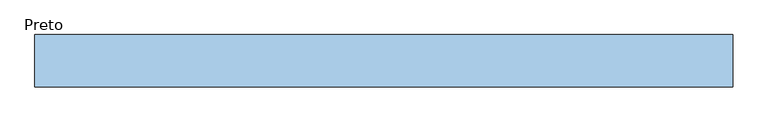
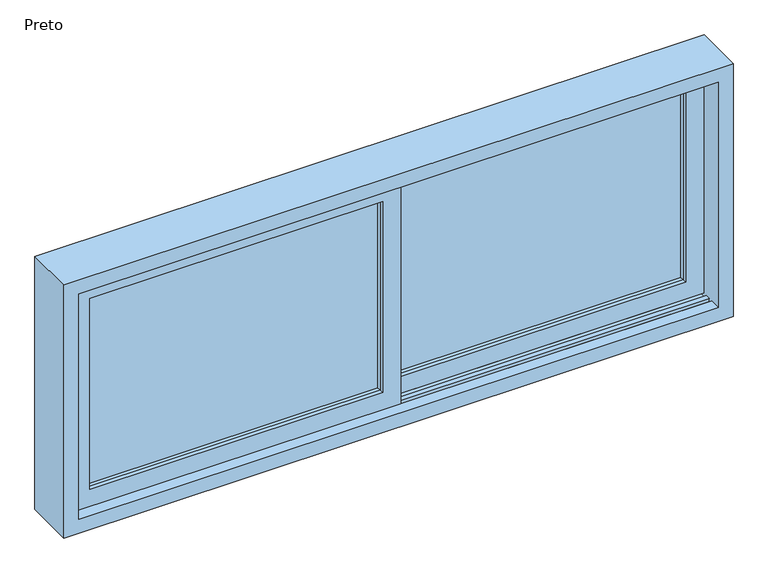
"""IFC4 building model written with IfcOpenShell, lengths in millimetres: window geometry, Blks_Cons Weiku_Janela de Correr 02 Folhas : Preto."""

from ifc_helpers import new_model, si_unit, frame, origin, place, context, project, spatial, polyline, outline, extrude, faceted_brep, source, transform, mapped, element, save


def preto_b46f8be3(model_context):
    return source(origin(), model_context, "Body", "SolidModel", [
        faceted_brep([(27.0, 13.0, 898.0), (27.0, 13.0, 1502.0), (27.0, 18.0, 1502.0), (27.0, 18.0, 898.0), (32.0, 18.0, 903.0), (32.0, 18.0, 1497.0), (902.0, 13.0, 1502.0), (902.0, 18.0, 1502.0), (897.0, 18.0, 1497.0), (902.0, 13.0, 898.0), (902.0, 18.0, 898.0), (897.0, 18.0, 903.0)], [[[0, 1, 2, 3]], [[4, 5, 1, 0]], [[1, 6, 7, 2]], [[5, 8, 6, 1]], [[6, 9, 10, 7]], [[8, 11, 9, 6]], [[3, 2, 7, 10], [5, 4, 11, 8]], [[9, 0, 3, 10]], [[11, 4, 0, 9]]]),
        faceted_brep([(902.0, 27.0, 898.0), (902.0, 27.0, 1502.0), (902.0, 22.0, 1502.0), (902.0, 22.0, 898.0), (27.0, 27.0, 1502.0), (27.0, 22.0, 1502.0), (27.0, 27.0, 898.0), (27.0, 22.0, 898.0), (897.0, 22.0, 1497.0), (897.0, 22.0, 903.0), (32.0, 22.0, 903.0), (32.0, 22.0, 1497.0)], [[[0, 1, 2, 3]], [[1, 4, 5, 2]], [[4, 6, 7, 5]], [[3, 2, 5, 7], [8, 9, 10, 11]], [[6, 0, 3, 7]], [[9, 8, 1, 0]], [[8, 11, 4, 1]], [[11, 10, 6, 4]], [[10, 9, 0, 6]]]),
        extrude(outline(polyline([(902.0, 22.0), (902.0, 18.0), (27.0, 18.0), (27.0, 22.0), (902.0, 22.0)])), frame((0.0, 0.0, 898.0), z_axis=(0.0, 0.0, 1.0), x_axis=(1.0, 0.0, 0.0)), (0.0, 0.0, 1.0), 604.0),
        extrude(outline(polyline([(844.0, 956.0), (1556.0, 956.0), (1556.0, -27.0), (844.0, -27.0), (844.0, 956.0)]), holes=[polyline([(1502.0, 27.0), (1502.0, 902.0), (898.0, 902.0), (898.0, 27.0), (1502.0, 27.0)])]), frame((0.0, 0.0, 0.0), z_axis=(0.0, 1.0, 0.0), x_axis=(0.0, 0.0, 1.0)), (0.0, 0.0, 1.0), 40.0),
        faceted_brep([(-902.0, -27.0, 898.0), (-902.0, -27.0, 1502.0), (-902.0, -22.0, 1502.0), (-902.0, -22.0, 898.0), (-897.0, -22.0, 903.0), (-897.0, -22.0, 1497.0), (-27.0, -27.0, 1502.0), (-27.0, -22.0, 1502.0), (-32.0, -22.0, 1497.0), (-27.0, -27.0, 898.0), (-27.0, -22.0, 898.0), (-32.0, -22.0, 903.0)], [[[0, 1, 2, 3]], [[4, 5, 1, 0]], [[1, 6, 7, 2]], [[5, 8, 6, 1]], [[6, 9, 10, 7]], [[8, 11, 9, 6]], [[3, 2, 7, 10], [5, 4, 11, 8]], [[9, 0, 3, 10]], [[11, 4, 0, 9]]]),
        faceted_brep([(-27.0, -13.0, 898.0), (-27.0, -13.0, 1502.0), (-27.0, -18.0, 1502.0), (-27.0, -18.0, 898.0), (-902.0, -13.0, 1502.0), (-902.0, -18.0, 1502.0), (-902.0, -13.0, 898.0), (-902.0, -18.0, 898.0), (-32.0, -18.0, 1497.0), (-32.0, -18.0, 903.0), (-897.0, -18.0, 903.0), (-897.0, -18.0, 1497.0)], [[[0, 1, 2, 3]], [[1, 4, 5, 2]], [[4, 6, 7, 5]], [[3, 2, 5, 7], [8, 9, 10, 11]], [[6, 0, 3, 7]], [[9, 8, 1, 0]], [[8, 11, 4, 1]], [[11, 10, 6, 4]], [[10, 9, 0, 6]]]),
        extrude(outline(polyline([(-27.0, -18.0), (-27.0, -22.0), (-902.0, -22.0), (-902.0, -18.0), (-27.0, -18.0)])), frame((0.0, 0.0, 898.0), z_axis=(0.0, 0.0, 1.0), x_axis=(1.0, 0.0, 0.0)), (0.0, 0.0, 1.0), 604.0),
        extrude(outline(polyline([(844.0, 27.0), (1556.0, 27.0), (1556.0, -956.0), (844.0, -956.0), (844.0, 27.0)]), holes=[polyline([(1502.0, -902.0), (1502.0, -27.0), (898.0, -27.0), (898.0, -902.0), (1502.0, -902.0)])]), frame((0.0, -40.0, 0.0), z_axis=(0.0, 1.0, 0.0), x_axis=(0.0, 0.0, 1.0)), (0.0, 0.0, 1.0), 40.0),
        faceted_brep([(956.0, -75.0, 844.0), (956.0, -40.0, 844.0), (-956.0, -40.0, 844.0), (-956.0, -75.0, 844.0), (-956.0, 75.0, 844.0), (-956.0, 40.0, 844.0), (956.0, 40.0, 844.0), (956.0, 75.0, 844.0), (-956.0, 13.0, 844.0), (956.0, 13.0, 844.0), (956.0, 27.0, 844.0), (-956.0, 27.0, 844.0), (-956.0, -27.0, 844.0), (956.0, -27.0, 844.0), (956.0, -13.0, 844.0), (-956.0, -13.0, 844.0), (1000.0, -75.0, 800.0), (1000.0, -75.0, 1600.0), (-1000.0, -75.0, 1600.0), (-1000.0, -75.0, 800.0), (-956.0, -75.0, 1556.0), (956.0, -75.0, 1556.0), (-956.0, -40.0, 834.0), (-956.0, -27.0, 834.0), (-956.0, -13.0, 834.0), (-956.0, 13.0, 834.0), (-956.0, 27.0, 834.0), (-956.0, 40.0, 834.0), (-956.0, 75.0, 1556.0), (-956.0, 40.0, 1556.0), (-956.0, 40.0, 1566.0), (-956.0, 27.0, 1566.0), (-956.0, 27.0, 1556.0), (-956.0, 13.0, 1556.0), (-956.0, 13.0, 1566.0), (-956.0, -13.0, 1566.0), (-956.0, -13.0, 1556.0), (-956.0, -27.0, 1556.0), (-956.0, -27.0, 1566.0), (-956.0, -40.0, 1566.0), (-956.0, -40.0, 1556.0), (956.0, -40.0, 834.0), (956.0, -40.0, 1556.0), (956.0, -40.0, 1566.0), (956.0, -27.0, 1566.0), (956.0, -27.0, 1556.0), (956.0, -13.0, 1556.0), (956.0, -13.0, 1566.0), (956.0, 13.0, 1566.0), (956.0, 13.0, 1556.0), (956.0, 27.0, 1556.0), (956.0, 27.0, 1566.0), (956.0, 40.0, 1566.0), (956.0, 40.0, 1556.0), (956.0, 75.0, 1556.0), (956.0, 40.0, 834.0), (956.0, 27.0, 834.0), (956.0, 13.0, 834.0), (956.0, -13.0, 834.0), (956.0, -27.0, 834.0), (-1000.0, 75.0, 800.0), (-1000.0, 75.0, 1600.0), (1000.0, 75.0, 1600.0), (1000.0, 75.0, 800.0)], [[[0, 1, 2, 3]], [[4, 5, 6, 7]], [[8, 9, 10, 11]], [[12, 13, 14, 15]], [[16, 17, 18, 19], [3, 20, 21, 0]], [[3, 2, 22, 23, 12, 15, 24, 25, 8, 11, 26, 27, 5, 4, 28, 29, 30, 31, 32, 33, 34, 35, 36, 37, 38, 39, 40, 20]], [[22, 2, 1, 41]], [[21, 42, 43, 44, 45, 46, 47, 48, 49, 50, 51, 52, 53, 54, 7, 6, 55, 56, 10, 9, 57, 58, 14, 13, 59, 41, 1, 0]], [[60, 61, 62, 63], [7, 54, 28, 4]], [[55, 6, 5, 27]], [[56, 26, 11, 10]], [[9, 8, 25, 57]], [[58, 24, 15, 14]], [[13, 12, 23, 59]], [[63, 62, 17, 16]], [[16, 19, 60, 63]], [[19, 18, 61, 60]], [[55, 27, 26, 56]], [[57, 25, 24, 58]], [[59, 23, 22, 41]], [[20, 40, 42, 21]], [[54, 53, 29, 28]], [[32, 50, 49, 33]], [[36, 46, 45, 37]], [[18, 17, 62, 61]], [[46, 36, 35, 47]], [[47, 35, 34, 48]], [[48, 34, 33, 49]], [[50, 32, 31, 51]], [[51, 31, 30, 52]], [[30, 29, 53, 52]], [[43, 42, 40, 39]], [[43, 39, 38, 44]], [[44, 38, 37, 45]]]),
    ])


if __name__ == "__main__":
    model = new_model("IFC4")
    model_context = context("Model", 3, world=origin())
    ifc_project = project(units=[si_unit("LENGTHUNIT", "METRE", prefix="MILLI")], contexts=[model_context])
    site = spatial("IfcSite", under=ifc_project)
    building = spatial("IfcBuilding", under=site)
    placement = place(None, origin())
    preto_shape = preto_b46f8be3(model_context)
    element("IfcWindow", 1, ObjectType="Blks_Cons Weiku_Janela de Correr 02 Folhas : Preto", at=placement, inside=building, context=model_context, shape_type="MappedRepresentation", body=[
        mapped(preto_shape, transform((0.0, 0.0, 0.0), x_axis=(1.0, 0.0, 0.0), y_axis=(0.0, 1.0, 0.0), z_axis=(0.0, 0.0, 1.0))),
    ])
    save(model, "model.ifc")

# Revit data of these elements
# Type "Blks_Cons Weiku_Janela de Correr 02 Folhas : Preto"
#   Type Mark = "J26"
#   Type Comments = "Janela de Correr 02 Folhas"
#   Manufacturer = "Weiku"
#   Created By / Criado Por / Creado por = "Blocks"
#   Author URL = "https://BlocksRvt.com/"
#   Author Contact = "info@blocksrvt.com"
#   Assembly Code = "Cons"
#   c [instance default] = 250 mm
#   b [instance default] = 912 mm
#   a [instance default] = 983 mm
#   Rough Width [instance default] = 2000 mm
#   Width [instance default] = 1912 mm
#   Espessura Folha [instance default] = 40 mm
#   Rough Height [instance default] = 1000 mm
#   Height [instance default] = 912 mm
#   Abertura Janela Equerda [instance default] = 0 mm
#   Abertura Janela Direita [instance default] = 0 mm
#   Vidro = .vidro_growarq
#   Vedação = Blks - Rubber - Black
#   Janela = Blks - Plastic - Black - Glazed
#   Wall Closure = (empty or 0)
# Element 1 (IfcWindow, "Blks_Cons Weiku_Janela de Correr 02 Folhas : Preto")
#   c = 200 mm
#   b = 712 mm
#   Rough Height = 800 mm
#   Height = 712 mm
#   Materials on its faces: "Blks - Plastic - Black - Glazed", "Blks - Rubber - Black", ".vidro_growarq"
# Materials
#   ".vidro_growarq": class "Vidro", colour RGB 200 215 215, transparency 0.6, Description = "Vidroverde", Cost = 0
#   "Blks - Rubber - Black": class "Paint/Coating", colour RGB 38 38 38, transparency 0, Cost = 0
#   "Blks - Plastic - Black - Glazed": class "Plastic", colour RGB 25 25 25, transparency 0, Cost = 0
